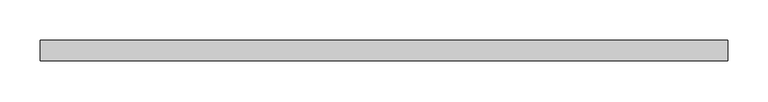
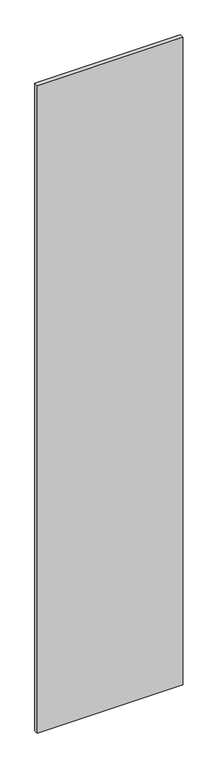
"""IFC4 building model written with IfcOpenShell, lengths in millimetres: plate geometry, 系统嵌板 : 玻璃."""

import ifcopenshell
import ifcopenshell.guid

model = None  # the IFC model being written
_history = None  # IfcOwnerHistory: only IFC2X3 demands one
_inside = {}  # id of a spatial element -> (the spatial element, [elements in it])
_under = {}  # id of a project, library or spatial element -> (it, [spatial elements below it])
_declared = {}  # id of a project -> (the project, [libraries it declares])
_typed = {}  # id of a type object -> (the type object, [elements of that type])
_made_of = {}  # id of a material, layer set ... -> (it, [elements and type objects made of it])


def new_model(schema):
    """Start an empty IFC model of exactly this schema.

    Asked for "IFC4X3", IfcOpenShell would pick the latest addendum, in which some entities
    have other attributes; the version numbers below select the first issue.
    IFC2X3 requires an IfcOwnerHistory on every rooted entity: one is made here for all.
    """
    global model, _history
    if schema == "IFC4X3":
        model = ifcopenshell.file(schema_version=(4, 3, 0, 0))
    else:
        model = ifcopenshell.file(schema=schema)
    _inside.clear()
    _under.clear()
    _declared.clear()
    _typed.clear()
    _made_of.clear()
    _history = None
    if model.schema == "IFC2X3":
        org = make("IfcOrganization", Name="unknown")
        user = make(
            "IfcPersonAndOrganization",
            ThePerson=make("IfcPerson", FamilyName="unknown"),
            TheOrganization=org,
        )
        app = make(
            "IfcApplication",
            ApplicationDeveloper=org,
            Version="unknown",
            ApplicationFullName="unknown",
            ApplicationIdentifier="unknown",
        )
        _history = make(
            "IfcOwnerHistory",
            OwningUser=user,
            OwningApplication=app,
            ChangeAction="ADDED",
            CreationDate=0,
        )
    return model


def make(cls, **values):
    """One entity of the class cls with the attributes given. An attribute that is None is left unset."""
    return model.create_entity(
        cls, **{name: value for name, value in values.items() if value is not None}
    )


def rooted(cls, **values):
    """An entity with a GlobalId (a new one), such as an element, a storey or a relation."""
    return make(cls, GlobalId=ifcopenshell.guid.new(), OwnerHistory=_history, **values)


def si_unit(unit_type, name, prefix=None):
    """IfcSIUnit, for example si_unit("LENGTHUNIT", "METRE", prefix="MILLI")."""
    return make("IfcSIUnit", UnitType=unit_type, Prefix=prefix, Name=name)


def assignment(units):
    """IfcUnitAssignment: the units of a project."""
    return None if units is None else make("IfcUnitAssignment", Units=units)


def point(xyz):
    """IfcCartesianPoint."""
    return None if xyz is None else make("IfcCartesianPoint", Coordinates=xyz)


def direction(xyz):
    """IfcDirection."""
    return None if xyz is None else make("IfcDirection", DirectionRatios=xyz)


def frame(location, z_axis=None, x_axis=None):
    """IfcAxis2Placement3D, a coordinate frame: its origin and axes. An axis left out is left unset."""
    return make(
        "IfcAxis2Placement3D",
        Location=point(location),
        Axis=direction(z_axis),
        RefDirection=direction(x_axis),
    )


def origin():
    """The frame at (0, 0, 0) with its axes left unset."""
    return frame((0.0, 0.0, 0.0))


def origin_with_axes():
    """The frame at (0, 0, 0) with the z axis (0, 0, 1) and the x axis (1, 0, 0) written out."""
    return frame((0.0, 0.0, 0.0), z_axis=(0.0, 0.0, 1.0), x_axis=(1.0, 0.0, 0.0))


def place(relative_to, where):
    """IfcLocalPlacement: puts the frame where relative to a parent placement (None: the world)."""
    return make(
        "IfcLocalPlacement", PlacementRelTo=relative_to, RelativePlacement=where
    )


def context(
    kind, dimensions, precision=None, world=None, true_north=None, identifier=None
):
    """IfcGeometricRepresentationContext, for example the 3D "Model" context."""
    return make(
        "IfcGeometricRepresentationContext",
        ContextIdentifier=identifier,
        ContextType=kind,
        CoordinateSpaceDimension=dimensions,
        Precision=precision,
        WorldCoordinateSystem=world,
        TrueNorth=true_north,
    )


def project(units=None, contexts=None):
    """IfcProject with its units and contexts."""
    return rooted(
        "IfcProject",
        Name="project",
        RepresentationContexts=contexts,
        UnitsInContext=assignment(units),
    )


def spatial(cls, under=None, at=None, **own):
    """A site, building, storey or space (cls), placed at a placement, below another one or the project."""
    s = rooted(cls, ObjectPlacement=at, **own)
    if under is not None:
        _under.setdefault(under.id(), (under, []))[1].append(s)
    return s


def polyline(points):
    """IfcPolyline through the points."""
    return make("IfcPolyline", Points=[point(p) for p in points])


def outline(outer, holes=None, kind="AREA"):
    """IfcArbitraryClosedProfileDef: a profile drawn as a closed curve; with holes, ...WithVoids."""
    if holes is None:
        return make("IfcArbitraryClosedProfileDef", ProfileType=kind, OuterCurve=outer)
    return make(
        "IfcArbitraryProfileDefWithVoids",
        ProfileType=kind,
        OuterCurve=outer,
        InnerCurves=holes,
    )


def extrude(swept, where, along, depth):
    """IfcExtrudedAreaSolid: the profile swept, set in the frame where, extruded along a direction by depth."""
    return make(
        "IfcExtrudedAreaSolid",
        SweptArea=swept,
        Position=where,
        ExtrudedDirection=direction(along),
        Depth=depth,
    )


def shape(context_of_items, identifier, shape_type, items):
    """IfcShapeRepresentation: the items that make up one representation, for example the "Body"."""
    return make(
        "IfcShapeRepresentation",
        ContextOfItems=context_of_items,
        RepresentationIdentifier=identifier,
        RepresentationType=shape_type,
        Items=items,
    )


def source(mapping_origin, context_of_items, identifier, shape_type, items):
    """IfcRepresentationMap: a shape defined once, which mapped items show again and again."""
    return make(
        "IfcRepresentationMap",
        MappingOrigin=mapping_origin,
        MappedRepresentation=shape(context_of_items, identifier, shape_type, items),
    )


def transform(
    local_origin,
    x_axis=None,
    y_axis=None,
    z_axis=None,
    scale=None,
    scale2=None,
    scale3=None,
    uniform=True,
):
    """IfcCartesianTransformationOperator3D, or its non-uniform kind. x_axis, y_axis, z_axis: its Axis1, 2, 3."""
    if uniform:
        return make(
            "IfcCartesianTransformationOperator3D",
            Axis1=direction(x_axis),
            Axis2=direction(y_axis),
            LocalOrigin=point(local_origin),
            Scale=scale,
            Axis3=direction(z_axis),
        )
    return make(
        "IfcCartesianTransformationOperator3DnonUniform",
        Axis1=direction(x_axis),
        Axis2=direction(y_axis),
        LocalOrigin=point(local_origin),
        Scale=scale,
        Axis3=direction(z_axis),
        Scale2=scale2,
        Scale3=scale3,
    )


def mapped(mapping_source, mapping_target):
    """IfcMappedItem: shows the shape of a source again, moved by a transform."""
    return make(
        "IfcMappedItem", MappingSource=mapping_source, MappingTarget=mapping_target
    )


def made_of(thing, what):
    """Note that an element or type object is made of a material, layer set ...; save() writes the relation."""
    if what is not None:
        _made_of.setdefault(what.id(), (what, []))[1].append(thing)
    return thing


def element(
    cls,
    number,
    at=None,
    inside=None,
    cuts=None,
    type_object=None,
    material=None,
    context=None,
    identifier="Body",
    shape_type=None,
    held_by="IfcProductDefinitionShape",
    body=None,
    shapes=None,
    **own,
):
    """One element of the class cls, such as IfcWall. Its Tag is "e" and its number.

    at: its placement. inside: the storey or other place that contains it. cuts: it is an
    opening in that element (IfcRelVoidsElement). A single representation is given by context,
    identifier, shape_type and body (its items); several are given by shapes. held_by: the class
    of the entity that holds the representations. save() writes the other relations.
    """
    e = rooted(cls, Tag="e%d" % number, ObjectPlacement=at, **own)
    if body is not None:
        shapes = [shape(context, identifier, shape_type, body)]
    if shapes is not None:
        e.Representation = make(held_by, Representations=shapes)
    if inside is not None:
        _inside.setdefault(inside.id(), (inside, []))[1].append(e)
    if cuts is not None:
        rooted(
            "IfcRelVoidsElement", RelatingBuildingElement=cuts, RelatedOpeningElement=e
        )
    if type_object is not None:
        _typed.setdefault(type_object.id(), (type_object, []))[1].append(e)
    return made_of(e, material)


def aggregate(whole, parts):
    """IfcRelAggregates: a whole, such as a stair, and the parts it consists of."""
    return rooted("IfcRelAggregates", RelatingObject=whole, RelatedObjects=parts)


def save(model, path):
    """Write the relations noted so far, then the file.

    IfcRelAggregates (storeys below a building ...), IfcRelContainedInSpatialStructure (elements
    in a storey), IfcRelDefinesByType, IfcRelAssociatesMaterial and IfcRelDeclares: one each for
    every whole, place, type object, material and project.
    """
    for whole, parts in _under.values():
        aggregate(whole, parts)
    for where, things in _inside.values():
        rooted(
            "IfcRelContainedInSpatialStructure",
            RelatedElements=things,
            RelatingStructure=where,
        )
    for kind, things in _typed.values():
        rooted("IfcRelDefinesByType", RelatedObjects=things, RelatingType=kind)
    for what, things in _made_of.values():
        rooted("IfcRelAssociatesMaterial", RelatedObjects=things, RelatingMaterial=what)
    for by, libraries in _declared.values():
        rooted("IfcRelDeclares", RelatingContext=by, RelatedDefinitions=libraries)
    model.write(path)


def plate_7a48b0fb(model_context):
    return source(origin(), model_context, "Body", "SweptSolid", [
        extrude(outline(polyline([(425.0, -12.5), (-425.0, -12.5), (-425.0, 12.5), (425.0, 12.5), (425.0, -12.5)])), origin_with_axes(), (0.0, 0.0, 1.0), 4000.0),
    ])


if __name__ == "__main__":
    model = new_model("IFC4")
    model_context = context("Model", 3, world=origin())
    ifc_project = project(units=[si_unit("LENGTHUNIT", "METRE", prefix="MILLI")], contexts=[model_context])
    site = spatial("IfcSite", under=ifc_project)
    building = spatial("IfcBuilding", under=site)
    placement = place(None, origin())
    plate_shape = plate_7a48b0fb(model_context)
    element("IfcPlate", 1, ObjectType="系统嵌板 : 玻璃", at=placement, inside=building, context=model_context, shape_type="MappedRepresentation", body=[
        mapped(plate_shape, transform((0.0, 0.0, 0.0), x_axis=(1.0, 0.0, 0.0), y_axis=(0.0, 1.0, 0.0), z_axis=(0.0, 0.0, 1.0))),
    ])
    save(model, "model.ifc")

# Revit data of these elements
# Type "系统嵌板 : 玻璃"
#   Construction Type Id = "GSP4R"
#   Analytic Construction = "1/8 英寸 Pilkington 单层玻璃"
#   Visual Light Transmittance = 0.9
#   Solar Heat Gain Coefficient = 0.86
#   Heat Transfer Coefficient (U) = 6.7069 W/(m²·K)
# Element 1 (IfcPlate, "系统嵌板 : 玻璃")
#   Materials on its faces: "玻璃"
# Materials
#   "玻璃": class "玻璃", colour RGB 0 128 192, transparency 0.9, Description = "钠钙玻璃", Cost = 0
